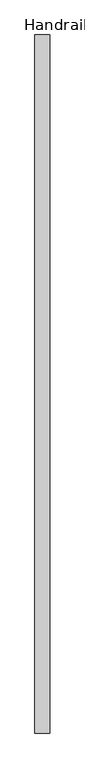
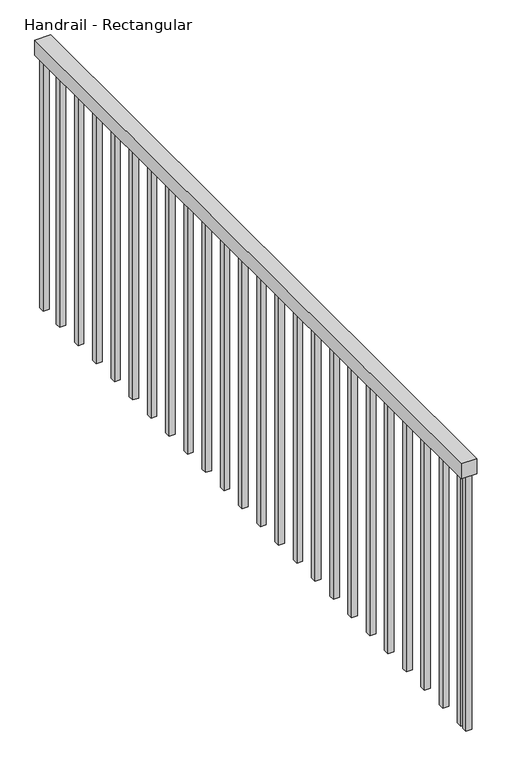
"""IFC4 building model written with IfcOpenShell, lengths in millimetres: railing geometry, Handrail - Rectangular."""

from ifc_helpers import new_model, si_unit, frame, origin, place, context, project, spatial, polyline, outline, extrude, source, transform, mapped, element, save


def handrail_rectangular_b6f31a4c(model_context):
    return source(origin(), model_context, "Body", "SweptSolid", [
        extrude(outline(polyline([(3383.9788909, 8595.8507146), (3434.7788909, 8595.8507146), (3434.7788909, 6220.8507146), (3383.9788909, 6220.8507146), (3383.9788909, 8595.8507146)])), frame((0.0, 0.0, 6654.4), z_axis=(0.0, 0.0, 1.0), x_axis=(1.0, 0.0, 0.0)), (0.0, 0.0, 1.0), 50.8),
        extrude(outline(polyline([(3399.8538909, 6268.5757146), (3418.9038909, 6268.5757146), (3418.9038909, 6249.5257146), (3399.8538909, 6249.5257146), (3399.8538909, 6268.5757146)])), frame((0.0, 0.0, 5790.8), z_axis=(0.0, 0.0, 1.0), x_axis=(1.0, 0.0, 0.0)), (0.0, 0.0, 1.0), 863.6),
        extrude(outline(polyline([(3399.8538909, 6370.1757146), (3418.9038909, 6370.1757146), (3418.9038909, 6351.1257146), (3399.8538909, 6351.1257146), (3399.8538909, 6370.1757146)])), frame((0.0, 0.0, 5790.8), z_axis=(0.0, 0.0, 1.0), x_axis=(1.0, 0.0, 0.0)), (0.0, 0.0, 1.0), 863.6),
        extrude(outline(polyline([(3399.8538909, 6471.7757146), (3418.9038909, 6471.7757146), (3418.9038909, 6452.7257146), (3399.8538909, 6452.7257146), (3399.8538909, 6471.7757146)])), frame((0.0, 0.0, 5790.8), z_axis=(0.0, 0.0, 1.0), x_axis=(1.0, 0.0, 0.0)), (0.0, 0.0, 1.0), 863.6),
        extrude(outline(polyline([(3399.8538909, 6573.3757146), (3418.9038909, 6573.3757146), (3418.9038909, 6554.3257146), (3399.8538909, 6554.3257146), (3399.8538909, 6573.3757146)])), frame((0.0, 0.0, 5790.8), z_axis=(0.0, 0.0, 1.0), x_axis=(1.0, 0.0, 0.0)), (0.0, 0.0, 1.0), 863.6),
        extrude(outline(polyline([(3399.8538909, 6674.9757146), (3418.9038909, 6674.9757146), (3418.9038909, 6655.9257146), (3399.8538909, 6655.9257146), (3399.8538909, 6674.9757146)])), frame((0.0, 0.0, 5790.8), z_axis=(0.0, 0.0, 1.0), x_axis=(1.0, 0.0, 0.0)), (0.0, 0.0, 1.0), 863.6),
        extrude(outline(polyline([(3399.8538909, 6776.5757146), (3418.9038909, 6776.5757146), (3418.9038909, 6757.5257146), (3399.8538909, 6757.5257146), (3399.8538909, 6776.5757146)])), frame((0.0, 0.0, 5790.8), z_axis=(0.0, 0.0, 1.0), x_axis=(1.0, 0.0, 0.0)), (0.0, 0.0, 1.0), 863.6),
        extrude(outline(polyline([(3399.8538909, 6878.1757146), (3418.9038909, 6878.1757146), (3418.9038909, 6859.1257146), (3399.8538909, 6859.1257146), (3399.8538909, 6878.1757146)])), frame((0.0, 0.0, 5790.8), z_axis=(0.0, 0.0, 1.0), x_axis=(1.0, 0.0, 0.0)), (0.0, 0.0, 1.0), 863.6),
        extrude(outline(polyline([(3399.8538909, 6979.7757146), (3418.9038909, 6979.7757146), (3418.9038909, 6960.7257146), (3399.8538909, 6960.7257146), (3399.8538909, 6979.7757146)])), frame((0.0, 0.0, 5790.8), z_axis=(0.0, 0.0, 1.0), x_axis=(1.0, 0.0, 0.0)), (0.0, 0.0, 1.0), 863.6),
        extrude(outline(polyline([(3399.8538909, 7081.3757146), (3418.9038909, 7081.3757146), (3418.9038909, 7062.3257146), (3399.8538909, 7062.3257146), (3399.8538909, 7081.3757146)])), frame((0.0, 0.0, 5790.8), z_axis=(0.0, 0.0, 1.0), x_axis=(1.0, 0.0, 0.0)), (0.0, 0.0, 1.0), 863.6),
        extrude(outline(polyline([(3399.8538909, 7182.9757146), (3418.9038909, 7182.9757146), (3418.9038909, 7163.9257146), (3399.8538909, 7163.9257146), (3399.8538909, 7182.9757146)])), frame((0.0, 0.0, 5790.8), z_axis=(0.0, 0.0, 1.0), x_axis=(1.0, 0.0, 0.0)), (0.0, 0.0, 1.0), 863.6),
        extrude(outline(polyline([(3399.8538909, 7284.5757146), (3418.9038909, 7284.5757146), (3418.9038909, 7265.5257146), (3399.8538909, 7265.5257146), (3399.8538909, 7284.5757146)])), frame((0.0, 0.0, 5790.8), z_axis=(0.0, 0.0, 1.0), x_axis=(1.0, 0.0, 0.0)), (0.0, 0.0, 1.0), 863.6),
        extrude(outline(polyline([(3399.8538909, 7386.1757146), (3418.9038909, 7386.1757146), (3418.9038909, 7367.1257146), (3399.8538909, 7367.1257146), (3399.8538909, 7386.1757146)])), frame((0.0, 0.0, 5790.8), z_axis=(0.0, 0.0, 1.0), x_axis=(1.0, 0.0, 0.0)), (0.0, 0.0, 1.0), 863.6),
        extrude(outline(polyline([(3399.8538909, 7487.7757146), (3418.9038909, 7487.7757146), (3418.9038909, 7468.7257146), (3399.8538909, 7468.7257146), (3399.8538909, 7487.7757146)])), frame((0.0, 0.0, 5790.8), z_axis=(0.0, 0.0, 1.0), x_axis=(1.0, 0.0, 0.0)), (0.0, 0.0, 1.0), 863.6),
        extrude(outline(polyline([(3399.8538909, 7589.3757146), (3418.9038909, 7589.3757146), (3418.9038909, 7570.3257146), (3399.8538909, 7570.3257146), (3399.8538909, 7589.3757146)])), frame((0.0, 0.0, 5790.8), z_axis=(0.0, 0.0, 1.0), x_axis=(1.0, 0.0, 0.0)), (0.0, 0.0, 1.0), 863.6),
        extrude(outline(polyline([(3399.8538909, 7690.9757146), (3418.9038909, 7690.9757146), (3418.9038909, 7671.9257146), (3399.8538909, 7671.9257146), (3399.8538909, 7690.9757146)])), frame((0.0, 0.0, 5790.8), z_axis=(0.0, 0.0, 1.0), x_axis=(1.0, 0.0, 0.0)), (0.0, 0.0, 1.0), 863.6),
        extrude(outline(polyline([(3399.8538909, 7792.5757146), (3418.9038909, 7792.5757146), (3418.9038909, 7773.5257146), (3399.8538909, 7773.5257146), (3399.8538909, 7792.5757146)])), frame((0.0, 0.0, 5790.8), z_axis=(0.0, 0.0, 1.0), x_axis=(1.0, 0.0, 0.0)), (0.0, 0.0, 1.0), 863.6),
        extrude(outline(polyline([(3399.8538909, 7894.1757146), (3418.9038909, 7894.1757146), (3418.9038909, 7875.1257146), (3399.8538909, 7875.1257146), (3399.8538909, 7894.1757146)])), frame((0.0, 0.0, 5790.8), z_axis=(0.0, 0.0, 1.0), x_axis=(1.0, 0.0, 0.0)), (0.0, 0.0, 1.0), 863.6),
        extrude(outline(polyline([(3399.8538909, 7995.7757146), (3418.9038909, 7995.7757146), (3418.9038909, 7976.7257146), (3399.8538909, 7976.7257146), (3399.8538909, 7995.7757146)])), frame((0.0, 0.0, 5790.8), z_axis=(0.0, 0.0, 1.0), x_axis=(1.0, 0.0, 0.0)), (0.0, 0.0, 1.0), 863.6),
        extrude(outline(polyline([(3399.8538909, 8097.3757146), (3418.9038909, 8097.3757146), (3418.9038909, 8078.3257146), (3399.8538909, 8078.3257146), (3399.8538909, 8097.3757146)])), frame((0.0, 0.0, 5790.8), z_axis=(0.0, 0.0, 1.0), x_axis=(1.0, 0.0, 0.0)), (0.0, 0.0, 1.0), 863.6),
        extrude(outline(polyline([(3399.8538909, 8198.9757146), (3418.9038909, 8198.9757146), (3418.9038909, 8179.9257146), (3399.8538909, 8179.9257146), (3399.8538909, 8198.9757146)])), frame((0.0, 0.0, 5790.8), z_axis=(0.0, 0.0, 1.0), x_axis=(1.0, 0.0, 0.0)), (0.0, 0.0, 1.0), 863.6),
        extrude(outline(polyline([(3399.8538909, 8300.5757146), (3418.9038909, 8300.5757146), (3418.9038909, 8281.5257146), (3399.8538909, 8281.5257146), (3399.8538909, 8300.5757146)])), frame((0.0, 0.0, 5790.8), z_axis=(0.0, 0.0, 1.0), x_axis=(1.0, 0.0, 0.0)), (0.0, 0.0, 1.0), 863.6),
        extrude(outline(polyline([(3399.8538909, 8402.1757146), (3418.9038909, 8402.1757146), (3418.9038909, 8383.1257146), (3399.8538909, 8383.1257146), (3399.8538909, 8402.1757146)])), frame((0.0, 0.0, 5790.8), z_axis=(0.0, 0.0, 1.0), x_axis=(1.0, 0.0, 0.0)), (0.0, 0.0, 1.0), 863.6),
        extrude(outline(polyline([(3399.8538909, 8503.7757146), (3418.9038909, 8503.7757146), (3418.9038909, 8484.7257146), (3399.8538909, 8484.7257146), (3399.8538909, 8503.7757146)])), frame((0.0, 0.0, 5790.8), z_axis=(0.0, 0.0, 1.0), x_axis=(1.0, 0.0, 0.0)), (0.0, 0.0, 1.0), 863.6),
        extrude(outline(polyline([(3399.8538909, 6239.9007146), (3418.9038909, 6239.9007146), (3418.9038909, 6220.8507146), (3399.8538909, 6220.8507146), (3399.8538909, 6239.9007146)])), frame((0.0, 0.0, 5790.8), z_axis=(0.0, 0.0, 1.0), x_axis=(1.0, 0.0, 0.0)), (0.0, 0.0, 1.0), 863.6),
        extrude(outline(polyline([(3399.8538909, 8595.8507146), (3418.9038909, 8595.8507146), (3418.9038909, 8576.8007146), (3399.8538909, 8576.8007146), (3399.8538909, 8595.8507146)])), frame((0.0, 0.0, 5790.8), z_axis=(0.0, 0.0, 1.0), x_axis=(1.0, 0.0, 0.0)), (0.0, 0.0, 1.0), 863.6),
    ])


if __name__ == "__main__":
    model = new_model("IFC4")
    model_context = context("Model", 3, world=origin())
    ifc_project = project(units=[si_unit("LENGTHUNIT", "METRE", prefix="MILLI")], contexts=[model_context])
    site = spatial("IfcSite", under=ifc_project)
    building = spatial("IfcBuilding", under=site)
    placement = place(None, origin())
    handrail_rectangular_shape = handrail_rectangular_b6f31a4c(model_context)
    element("IfcRailing", 1, ObjectType="Handrail - Rectangular", at=placement, inside=building, context=model_context, shape_type="MappedRepresentation", body=[
        mapped(handrail_rectangular_shape, transform((0.0, 0.0, 0.0), x_axis=(1.0, 0.0, 0.0), y_axis=(0.0, 1.0, 0.0), z_axis=(0.0, 0.0, 1.0))),
    ])
    save(model, "model.ifc")
